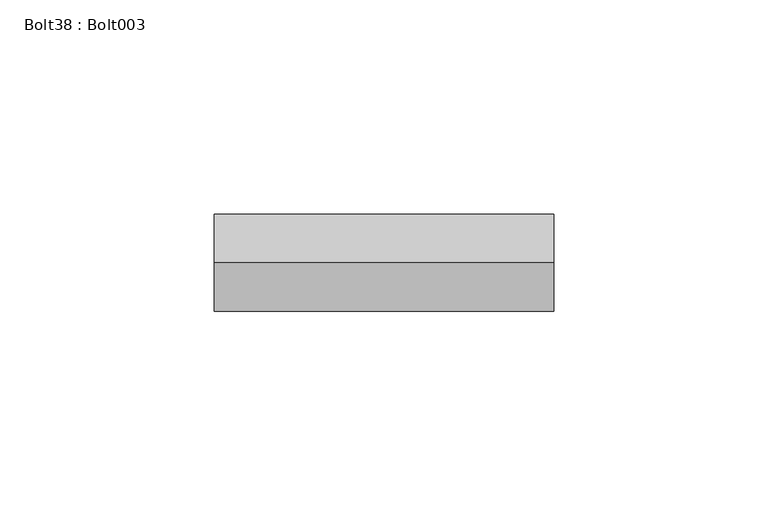
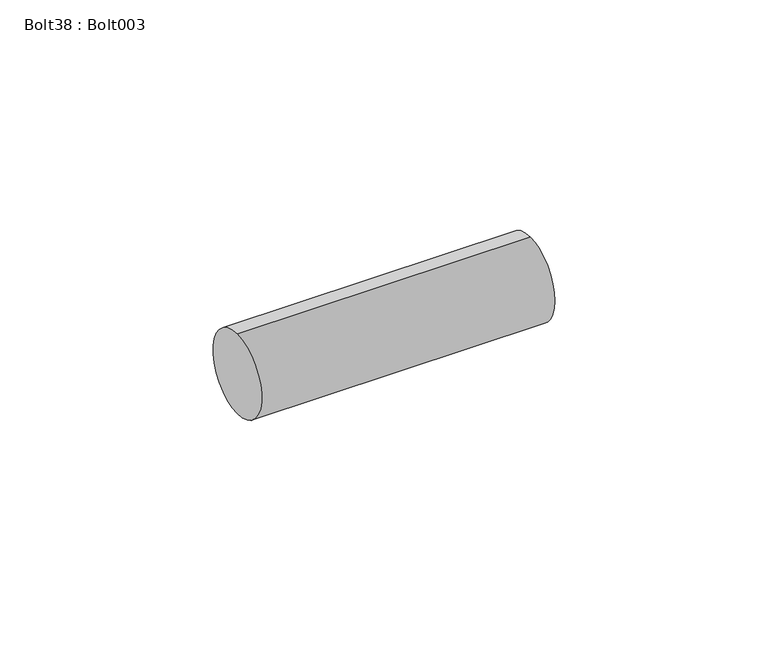
"""IFC4 building model written with IfcOpenShell, lengths in millimetres: proxy geometry, Bolt38 : Bolt003."""

from ifc_helpers import new_model, si_unit, point, frame, frame_2d, origin, place, context, project, spatial, circle_curve, trimmed, segment, composite_curve, outline, extrude, source, transform, mapped, element, save


def bolt38_bolt003_f2b5b441(model_context):
    return source(origin(), model_context, "Body", "SweptSolid", [
        extrude(outline(composite_curve([segment(trimmed(circle_curve(frame_2d((1985.8304801, 40070.0545241)), 11.4045168), [point((1985.8304801, 40058.6500073))], [point((1985.8304801, 40081.4590409))], False, "CARTESIAN"), True, "CONTINUOUS"), segment(trimmed(circle_curve(frame_2d((1985.8304801, 40070.0545241)), 11.4045168), [point((1985.8304801, 40081.4590409))], [point((1985.8304801, 40058.6500073))], False, "CARTESIAN"), True, "CONTINUOUS")], self_intersect=False)), frame((10265.0890809, 0.0, 0.0), z_axis=(1.0, 0.0, 0.0), x_axis=(0.0, 1.0, 0.0)), (0.0, 0.0, 1.0), 79.375),
    ])


if __name__ == "__main__":
    model = new_model("IFC4")
    model_context = context("Model", 3, world=origin())
    ifc_project = project(units=[si_unit("LENGTHUNIT", "METRE", prefix="MILLI")], contexts=[model_context])
    site = spatial("IfcSite", under=ifc_project)
    building = spatial("IfcBuilding", under=site)
    placement = place(None, origin())
    bolt38_bolt003_shape = bolt38_bolt003_f2b5b441(model_context)
    element("IfcBuildingElementProxy", 1, Name="Bolt38 : Bolt003", ObjectType="Bolt38 : Bolt003", at=placement, inside=building, context=model_context, shape_type="MappedRepresentation", body=[
        mapped(bolt38_bolt003_shape, transform((0.0, 0.0, 0.0), x_axis=(1.0, 0.0, 0.0), y_axis=(0.0, 1.0, 0.0), z_axis=(0.0, 0.0, 1.0))),
    ])
    save(model, "model.ifc")

# Revit data of these elements
# Type "Bolt38 : Bolt003"
#   NameOverride = "Bolt003"
# Element 1 (IfcBuildingElementProxy, "Bolt38 : Bolt003")
#   Materials on its faces: "STEEL ANGLE AND ANCHOR BOLT (SEE STRUCT. DWGS)"
# Materials
#   "STEEL ANGLE AND ANCHOR BOLT (SEE STRUCT. DWGS)": class "Unassigned", colour RGB 128 128 128, transparency 0, Cost = 0
